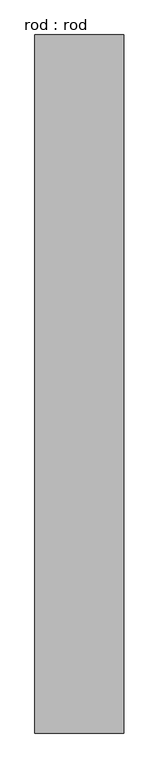
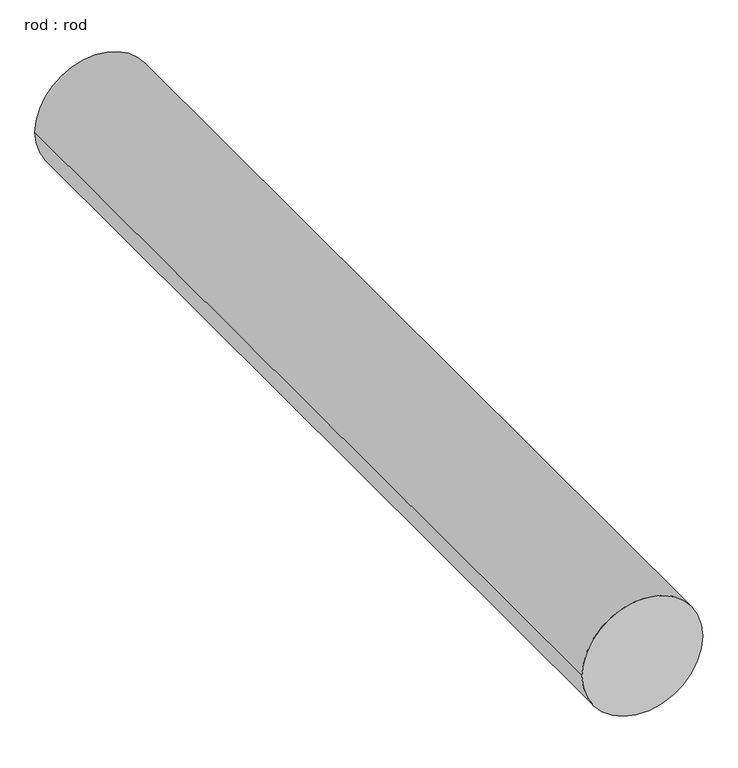
"""IFC4 building model written with IfcOpenShell, lengths in millimetres: proxy geometry, rod : rod."""

from ifc_helpers import new_model, si_unit, point, frame, frame_2d, origin, place, context, project, spatial, circle_curve, trimmed, segment, composite_curve, outline, extrude, source, transform, mapped, element, save


def rod_rod_69e50361(model_context):
    return source(origin(), model_context, "Body", "SweptSolid", [
        extrude(outline(composite_curve([segment(trimmed(circle_curve(frame_2d((0.0108462, 0.0)), 200.0), [point((0.0108462, 200.0))], [point((0.0108462, -200.0))], False, "CARTESIAN"), True, "CONTINUOUS"), segment(trimmed(circle_curve(frame_2d((0.0108462, 0.0)), 200.0), [point((0.0108462, -200.0))], [point((0.0108462, 200.0))], False, "CARTESIAN"), True, "CONTINUOUS")], self_intersect=False)), frame((0.0, 2522.7286153, 0.0), z_axis=(0.0, 1.0, 0.0), x_axis=(0.0, 0.0, 1.0)), (0.0, 0.0, 1.0), 3140.0),
    ])


if __name__ == "__main__":
    model = new_model("IFC4")
    model_context = context("Model", 3, world=origin())
    ifc_project = project(units=[si_unit("LENGTHUNIT", "METRE", prefix="MILLI")], contexts=[model_context])
    site = spatial("IfcSite", under=ifc_project)
    building = spatial("IfcBuilding", under=site)
    placement = place(None, origin())
    rod_rod_shape = rod_rod_69e50361(model_context)
    element("IfcBuildingElementProxy", 1, Name="rod : rod", ObjectType="rod : rod", at=placement, inside=building, context=model_context, shape_type="MappedRepresentation", body=[
        mapped(rod_rod_shape, transform((0.0, 0.0, 0.0), x_axis=(1.0, 0.0, 0.0), y_axis=(0.0, 1.0, 0.0), z_axis=(0.0, 0.0, 1.0))),
    ])
    save(model, "model.ifc")

# Revit data of these elements
# Type "rod : rod"
#   Default Elevation = 0
